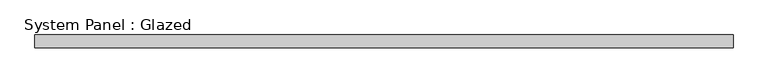
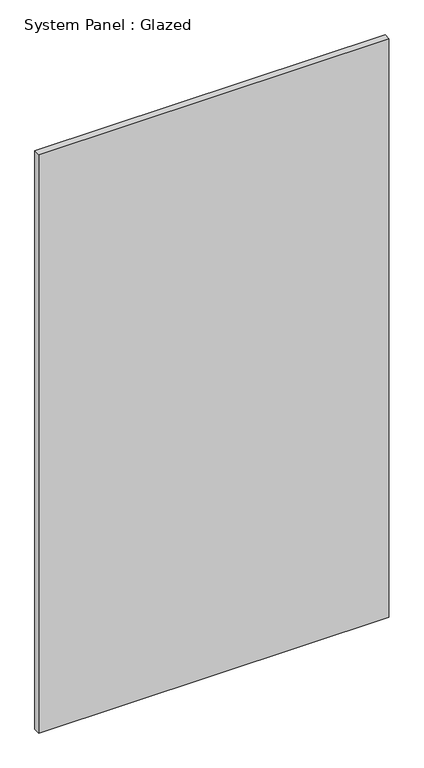
"""IFC4 building model written with IfcOpenShell, lengths in millimetres: plate geometry, System Panel : Glazed."""

from ifc_helpers import new_model, si_unit, origin, origin_with_axes, place, context, project, spatial, polyline, outline, extrude, source, transform, mapped, element, save


def system_panel_glazed_fd28fc1d(model_context):
    return source(origin(), model_context, "Body", "SweptSolid", [
        extrude(outline(polyline([(687.25, 24.5), (-687.25, 24.5), (-687.25, 49.5), (687.25, 49.5), (687.25, 24.5)])), origin_with_axes(), (0.0, 0.0, 1.0), 2400.0),
    ])


if __name__ == "__main__":
    model = new_model("IFC4")
    model_context = context("Model", 3, world=origin())
    ifc_project = project(units=[si_unit("LENGTHUNIT", "METRE", prefix="MILLI")], contexts=[model_context])
    site = spatial("IfcSite", under=ifc_project)
    building = spatial("IfcBuilding", under=site)
    placement = place(None, origin())
    system_panel_glazed_shape = system_panel_glazed_fd28fc1d(model_context)
    element("IfcPlate", 1, ObjectType="System Panel : Glazed", at=placement, inside=building, context=model_context, shape_type="MappedRepresentation", body=[
        mapped(system_panel_glazed_shape, transform((0.0, 0.0, 0.0), x_axis=(1.0, 0.0, 0.0), y_axis=(0.0, 1.0, 0.0), z_axis=(0.0, 0.0, 1.0))),
    ])
    save(model, "model.ifc")

# Revit data of these elements
# Element 1 (IfcPlate, "System Panel : Glazed")
#   Materials on its faces: "Glass"
# Materials
#   "Glass": class "Glass", colour RGB 218 227 224, transparency 0.85, Description = "Soda Lime Glass", Cost = 0
